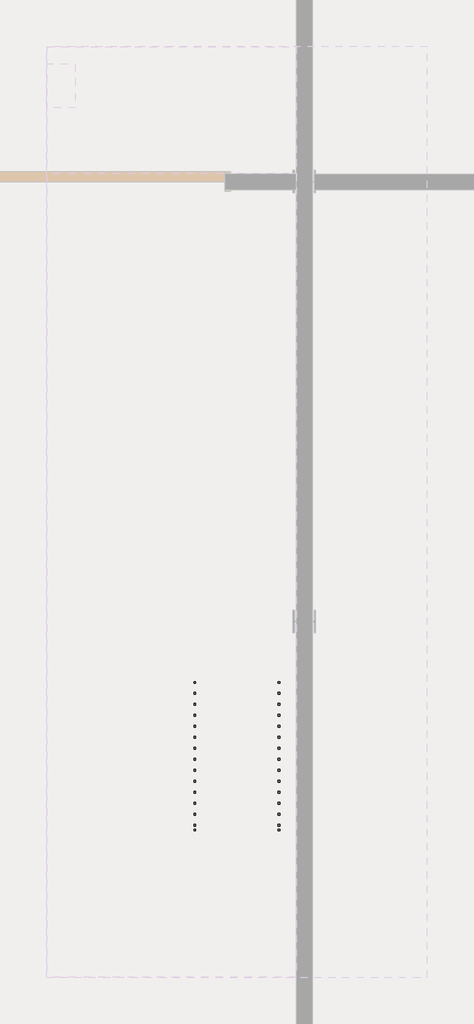
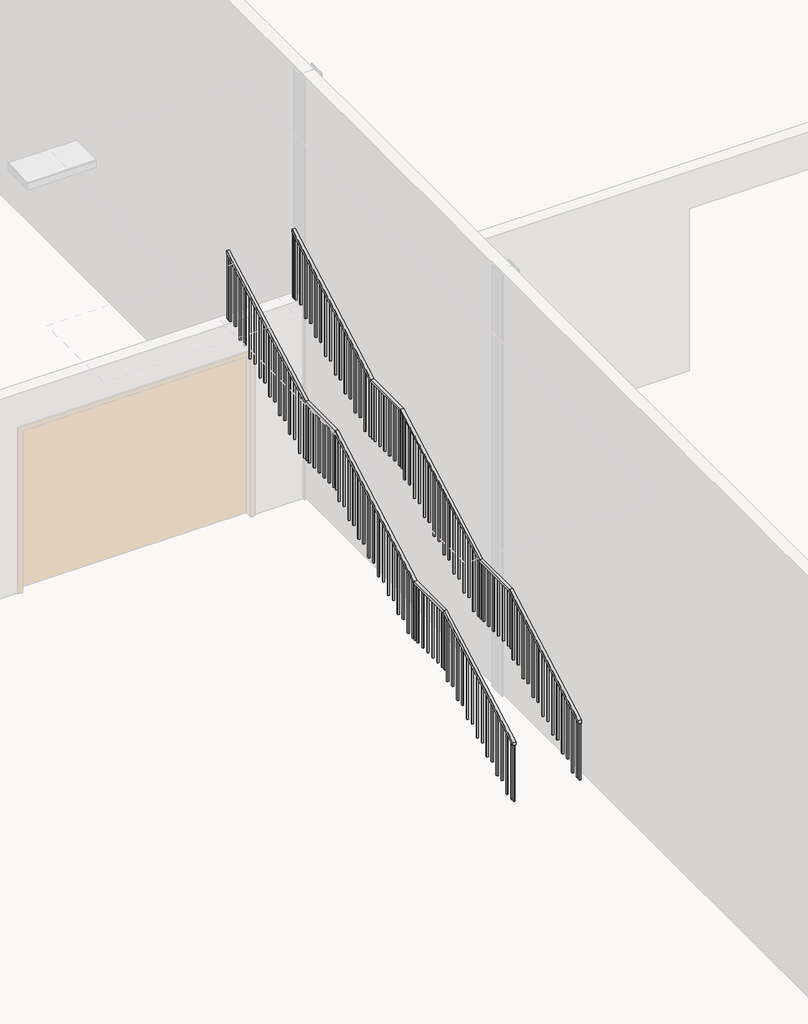
# One storey, part 8 of 13: 2 railings.
"""IFC4 building model written with IfcOpenShell, lengths in millimetres."""

from ifc_helpers import new_model, si_unit, frame, origin, place, context, project, spatial, polyline, outline, extrude, faceted_brep, element, save

model = new_model("IFC4")

# Units and contexts
model_context = context("Model", 3, world=origin())
ifc_project = project(units=[si_unit("LENGTHUNIT", "METRE", prefix="MILLI")], contexts=[model_context])

# Site, building, storey
site = spatial("IfcSite", under=ifc_project)
building = spatial("IfcBuilding", under=site)
storey = spatial("IfcBuildingStorey", under=building, Name="L0 - Ground Floor (Shadows On)", Elevation=0.0)

# Railings
placement = place(None, origin())
element("IfcRailing", 1, ObjectType="1100mm", at=placement, inside=storey, context=model_context, shape_type="SolidModel", body=[
    faceted_brep([(10487.9745537, -13916.6257726, 1266.6666667), (10487.9745537, -13916.6257726, 1209.4687214), (10537.9745537, -13916.6257726, 1209.4687214), (10537.9745537, -13916.6257726, 1266.6666667), (10487.9745537, -11816.6257726, 2433.3333333), (10487.9745537, -11803.6694712, 2383.3333333), (10537.9745537, -11803.6694712, 2383.3333333), (10537.9745537, -11816.6257726, 2433.3333333), (10487.9745537, -10916.6257726, 2433.3333333), (10487.9745537, -10903.6694712, 2383.3333333), (10537.9745537, -10903.6694712, 2383.3333333), (10537.9745537, -10916.6257726, 2433.3333333), (10487.9745537, -8516.6257726, 3766.6666667), (10487.9745537, -8503.6694712, 3716.6666667), (10537.9745537, -8503.6694712, 3716.6666667), (10537.9745537, -8516.6257726, 3766.6666667), (10487.9745537, -7616.6257726, 3766.6666667), (10487.9745537, -7603.6694712, 3716.6666667), (10537.9745537, -7603.6694712, 3716.6666667), (10537.9745537, -7616.6257726, 3766.6666667), (10487.9745537, -5216.6257726, 5100.0), (10537.9745537, -5216.6257726, 5100.0), (10537.9745537, -5216.6257726, 5042.8020548), (10487.9745537, -5216.6257726, 5042.8020548)], [[[0, 1, 2, 3]], [[1, 0, 4, 5]], [[2, 1, 5, 6]], [[3, 2, 6, 7]], [[0, 3, 7, 4]], [[5, 4, 8, 9]], [[6, 5, 9, 10]], [[7, 6, 10, 11]], [[4, 7, 11, 8]], [[9, 8, 12, 13]], [[10, 9, 13, 14]], [[11, 10, 14, 15]], [[8, 11, 15, 12]], [[13, 12, 16, 17]], [[14, 13, 17, 18]], [[15, 14, 18, 19]], [[12, 15, 19, 16]], [[20, 21, 22, 23]], [[17, 16, 20, 23]], [[18, 17, 23, 22]], [[19, 18, 22, 21]], [[16, 19, 21, 20]]]),
    extrude(outline(polyline([(-5304.1257726, 3833.3333333), (-5304.1257726, 4994.1909437), (-5279.1257726, 5008.0798326), (-5279.1257726, 3833.3333333), (-5304.1257726, 3833.3333333)])), frame((10500.4745537, 0.0, 0.0), z_axis=(1.0, 0.0, 0.0), x_axis=(0.0, 1.0, 0.0)), (0.0, 0.0, 1.0), 25.0),
    extrude(outline(polyline([(-5454.1257726, 3833.3333333), (-5454.1257726, 4910.8576103), (-5429.1257726, 4924.7464992), (-5429.1257726, 3833.3333333), (-5454.1257726, 3833.3333333)])), frame((10500.4745537, 0.0, 0.0), z_axis=(1.0, 0.0, 0.0), x_axis=(0.0, 1.0, 0.0)), (0.0, 0.0, 1.0), 25.0),
    extrude(outline(polyline([(-5604.1257726, 3666.6666667), (-5604.1257726, 4827.524277), (-5579.1257726, 4841.4131659), (-5579.1257726, 3666.6666667), (-5604.1257726, 3666.6666667)])), frame((10500.4745537, 0.0, 0.0), z_axis=(1.0, 0.0, 0.0), x_axis=(0.0, 1.0, 0.0)), (0.0, 0.0, 1.0), 25.0),
    extrude(outline(polyline([(-5754.1257726, 3666.6666667), (-5754.1257726, 4744.1909437), (-5729.1257726, 4758.0798326), (-5729.1257726, 3666.6666667), (-5754.1257726, 3666.6666667)])), frame((10500.4745537, 0.0, 0.0), z_axis=(1.0, 0.0, 0.0), x_axis=(0.0, 1.0, 0.0)), (0.0, 0.0, 1.0), 25.0),
    extrude(outline(polyline([(-5904.1257726, 3500.0), (-5904.1257726, 4660.8576103), (-5879.1257726, 4674.7464992), (-5879.1257726, 3500.0), (-5904.1257726, 3500.0)])), frame((10500.4745537, 0.0, 0.0), z_axis=(1.0, 0.0, 0.0), x_axis=(0.0, 1.0, 0.0)), (0.0, 0.0, 1.0), 25.0),
    extrude(outline(polyline([(-6054.1257726, 3500.0), (-6054.1257726, 4577.524277), (-6029.1257726, 4591.4131659), (-6029.1257726, 3500.0), (-6054.1257726, 3500.0)])), frame((10500.4745537, 0.0, 0.0), z_axis=(1.0, 0.0, 0.0), x_axis=(0.0, 1.0, 0.0)), (0.0, 0.0, 1.0), 25.0),
    extrude(outline(polyline([(-6204.1257726, 3333.3333333), (-6204.1257726, 4494.1909437), (-6179.1257726, 4508.0798326), (-6179.1257726, 3333.3333333), (-6204.1257726, 3333.3333333)])), frame((10500.4745537, 0.0, 0.0), z_axis=(1.0, 0.0, 0.0), x_axis=(0.0, 1.0, 0.0)), (0.0, 0.0, 1.0), 25.0),
    extrude(outline(polyline([(-6354.1257726, 3333.3333333), (-6354.1257726, 4410.8576103), (-6329.1257726, 4424.7464992), (-6329.1257726, 3333.3333333), (-6354.1257726, 3333.3333333)])), frame((10500.4745537, 0.0, 0.0), z_axis=(1.0, 0.0, 0.0), x_axis=(0.0, 1.0, 0.0)), (0.0, 0.0, 1.0), 25.0),
    extrude(outline(polyline([(-6504.1257726, 3166.6666667), (-6504.1257726, 4327.524277), (-6479.1257726, 4341.4131659), (-6479.1257726, 3166.6666667), (-6504.1257726, 3166.6666667)])), frame((10500.4745537, 0.0, 0.0), z_axis=(1.0, 0.0, 0.0), x_axis=(0.0, 1.0, 0.0)), (0.0, 0.0, 1.0), 25.0),
    extrude(outline(polyline([(-6654.1257726, 3166.6666667), (-6654.1257726, 4244.1909437), (-6629.1257726, 4258.0798326), (-6629.1257726, 3166.6666667), (-6654.1257726, 3166.6666667)])), frame((10500.4745537, 0.0, 0.0), z_axis=(1.0, 0.0, 0.0), x_axis=(0.0, 1.0, 0.0)), (0.0, 0.0, 1.0), 25.0),
    extrude(outline(polyline([(-6804.1257726, 3000.0), (-6804.1257726, 4160.8576103), (-6779.1257726, 4174.7464992), (-6779.1257726, 3000.0), (-6804.1257726, 3000.0)])), frame((10500.4745537, 0.0, 0.0), z_axis=(1.0, 0.0, 0.0), x_axis=(0.0, 1.0, 0.0)), (0.0, 0.0, 1.0), 25.0),
    extrude(outline(polyline([(-6954.1257726, 3000.0), (-6954.1257726, 4077.524277), (-6929.1257726, 4091.4131659), (-6929.1257726, 3000.0), (-6954.1257726, 3000.0)])), frame((10500.4745537, 0.0, 0.0), z_axis=(1.0, 0.0, 0.0), x_axis=(0.0, 1.0, 0.0)), (0.0, 0.0, 1.0), 25.0),
    extrude(outline(polyline([(-7104.1257726, 2833.3333333), (-7104.1257726, 3994.1909437), (-7079.1257726, 4008.0798326), (-7079.1257726, 2833.3333333), (-7104.1257726, 2833.3333333)])), frame((10500.4745537, 0.0, 0.0), z_axis=(1.0, 0.0, 0.0), x_axis=(0.0, 1.0, 0.0)), (0.0, 0.0, 1.0), 25.0),
    extrude(outline(polyline([(-7254.1257726, 2833.3333333), (-7254.1257726, 3910.8576103), (-7229.1257726, 3924.7464992), (-7229.1257726, 2833.3333333), (-7254.1257726, 2833.3333333)])), frame((10500.4745537, 0.0, 0.0), z_axis=(1.0, 0.0, 0.0), x_axis=(0.0, 1.0, 0.0)), (0.0, 0.0, 1.0), 25.0),
    extrude(outline(polyline([(-7404.1257726, 2666.6666667), (-7404.1257726, 3827.524277), (-7379.1257726, 3841.4131659), (-7379.1257726, 2666.6666667), (-7404.1257726, 2666.6666667)])), frame((10500.4745537, 0.0, 0.0), z_axis=(1.0, 0.0, 0.0), x_axis=(0.0, 1.0, 0.0)), (0.0, 0.0, 1.0), 25.0),
    extrude(outline(polyline([(-7554.1257726, 2666.6666667), (-7554.1257726, 3744.1909437), (-7529.1257726, 3758.0798326), (-7529.1257726, 2666.6666667), (-7554.1257726, 2666.6666667)])), frame((10500.4745537, 0.0, 0.0), z_axis=(1.0, 0.0, 0.0), x_axis=(0.0, 1.0, 0.0)), (0.0, 0.0, 1.0), 25.0),
    extrude(outline(polyline([(10525.4745537, -7704.1257726), (10500.4745537, -7704.1257726), (10500.4745537, -7679.1257726), (10525.4745537, -7679.1257726), (10525.4745537, -7704.1257726)])), frame((0.0, 0.0, 2666.6666667), z_axis=(0.0, 0.0, 1.0), x_axis=(1.0, 0.0, 0.0)), (0.0, 0.0, 1.0), 1050.0),
    extrude(outline(polyline([(10525.4745537, -7854.1257726), (10500.4745537, -7854.1257726), (10500.4745537, -7829.1257726), (10525.4745537, -7829.1257726), (10525.4745537, -7854.1257726)])), frame((0.0, 0.0, 2666.6666667), z_axis=(0.0, 0.0, 1.0), x_axis=(1.0, 0.0, 0.0)), (0.0, 0.0, 1.0), 1050.0),
    extrude(outline(polyline([(10525.4745537, -8004.1257726), (10500.4745537, -8004.1257726), (10500.4745537, -7979.1257726), (10525.4745537, -7979.1257726), (10525.4745537, -8004.1257726)])), frame((0.0, 0.0, 2666.6666667), z_axis=(0.0, 0.0, 1.0), x_axis=(1.0, 0.0, 0.0)), (0.0, 0.0, 1.0), 1050.0),
    extrude(outline(polyline([(10525.4745537, -8154.1257726), (10500.4745537, -8154.1257726), (10500.4745537, -8129.1257726), (10525.4745537, -8129.1257726), (10525.4745537, -8154.1257726)])), frame((0.0, 0.0, 2666.6666667), z_axis=(0.0, 0.0, 1.0), x_axis=(1.0, 0.0, 0.0)), (0.0, 0.0, 1.0), 1050.0),
    extrude(outline(polyline([(10525.4745537, -8304.1257726), (10500.4745537, -8304.1257726), (10500.4745537, -8279.1257726), (10525.4745537, -8279.1257726), (10525.4745537, -8304.1257726)])), frame((0.0, 0.0, 2666.6666667), z_axis=(0.0, 0.0, 1.0), x_axis=(1.0, 0.0, 0.0)), (0.0, 0.0, 1.0), 1050.0),
    extrude(outline(polyline([(10525.4745537, -8454.1257726), (10500.4745537, -8454.1257726), (10500.4745537, -8429.1257726), (10525.4745537, -8429.1257726), (10525.4745537, -8454.1257726)])), frame((0.0, 0.0, 2666.6666667), z_axis=(0.0, 0.0, 1.0), x_axis=(1.0, 0.0, 0.0)), (0.0, 0.0, 1.0), 1050.0),
    extrude(outline(polyline([(-8604.1257726, 2500.0), (-8604.1257726, 3660.8576103), (-8579.1257726, 3674.7464992), (-8579.1257726, 2500.0), (-8604.1257726, 2500.0)])), frame((10500.4745537, 0.0, 0.0), z_axis=(1.0, 0.0, 0.0), x_axis=(0.0, 1.0, 0.0)), (0.0, 0.0, 1.0), 25.0),
    extrude(outline(polyline([(-8754.1257726, 2500.0), (-8754.1257726, 3577.524277), (-8729.1257726, 3591.4131659), (-8729.1257726, 2500.0), (-8754.1257726, 2500.0)])), frame((10500.4745537, 0.0, 0.0), z_axis=(1.0, 0.0, 0.0), x_axis=(0.0, 1.0, 0.0)), (0.0, 0.0, 1.0), 25.0),
    extrude(outline(polyline([(-8904.1257726, 2333.3333333), (-8904.1257726, 3494.1909437), (-8879.1257726, 3508.0798326), (-8879.1257726, 2333.3333333), (-8904.1257726, 2333.3333333)])), frame((10500.4745537, 0.0, 0.0), z_axis=(1.0, 0.0, 0.0), x_axis=(0.0, 1.0, 0.0)), (0.0, 0.0, 1.0), 25.0),
    extrude(outline(polyline([(-9054.1257726, 2333.3333333), (-9054.1257726, 3410.8576103), (-9029.1257726, 3424.7464992), (-9029.1257726, 2333.3333333), (-9054.1257726, 2333.3333333)])), frame((10500.4745537, 0.0, 0.0), z_axis=(1.0, 0.0, 0.0), x_axis=(0.0, 1.0, 0.0)), (0.0, 0.0, 1.0), 25.0),
    extrude(outline(polyline([(-9204.1257726, 2166.6666667), (-9204.1257726, 3327.524277), (-9179.1257726, 3341.4131659), (-9179.1257726, 2166.6666667), (-9204.1257726, 2166.6666667)])), frame((10500.4745537, 0.0, 0.0), z_axis=(1.0, 0.0, 0.0), x_axis=(0.0, 1.0, 0.0)), (0.0, 0.0, 1.0), 25.0),
    extrude(outline(polyline([(-9354.1257726, 2166.6666667), (-9354.1257726, 3244.1909437), (-9329.1257726, 3258.0798326), (-9329.1257726, 2166.6666667), (-9354.1257726, 2166.6666667)])), frame((10500.4745537, 0.0, 0.0), z_axis=(1.0, 0.0, 0.0), x_axis=(0.0, 1.0, 0.0)), (0.0, 0.0, 1.0), 25.0),
    extrude(outline(polyline([(-9504.1257726, 2000.0), (-9504.1257726, 3160.8576103), (-9479.1257726, 3174.7464992), (-9479.1257726, 2000.0), (-9504.1257726, 2000.0)])), frame((10500.4745537, 0.0, 0.0), z_axis=(1.0, 0.0, 0.0), x_axis=(0.0, 1.0, 0.0)), (0.0, 0.0, 1.0), 25.0),
    extrude(outline(polyline([(-9654.1257726, 2000.0), (-9654.1257726, 3077.524277), (-9629.1257726, 3091.4131659), (-9629.1257726, 2000.0), (-9654.1257726, 2000.0)])), frame((10500.4745537, 0.0, 0.0), z_axis=(1.0, 0.0, 0.0), x_axis=(0.0, 1.0, 0.0)), (0.0, 0.0, 1.0), 25.0),
    extrude(outline(polyline([(-9804.1257726, 1833.3333333), (-9804.1257726, 2994.1909437), (-9779.1257726, 3008.0798326), (-9779.1257726, 1833.3333333), (-9804.1257726, 1833.3333333)])), frame((10500.4745537, 0.0, 0.0), z_axis=(1.0, 0.0, 0.0), x_axis=(0.0, 1.0, 0.0)), (0.0, 0.0, 1.0), 25.0),
    extrude(outline(polyline([(-9954.1257726, 1833.3333333), (-9954.1257726, 2910.8576103), (-9929.1257726, 2924.7464992), (-9929.1257726, 1833.3333333), (-9954.1257726, 1833.3333333)])), frame((10500.4745537, 0.0, 0.0), z_axis=(1.0, 0.0, 0.0), x_axis=(0.0, 1.0, 0.0)), (0.0, 0.0, 1.0), 25.0),
    extrude(outline(polyline([(-10104.1257726, 1666.6666667), (-10104.1257726, 2827.524277), (-10079.1257726, 2841.4131659), (-10079.1257726, 1666.6666667), (-10104.1257726, 1666.6666667)])), frame((10500.4745537, 0.0, 0.0), z_axis=(1.0, 0.0, 0.0), x_axis=(0.0, 1.0, 0.0)), (0.0, 0.0, 1.0), 25.0),
    extrude(outline(polyline([(-10254.1257726, 1666.6666667), (-10254.1257726, 2744.1909437), (-10229.1257726, 2758.0798326), (-10229.1257726, 1666.6666667), (-10254.1257726, 1666.6666667)])), frame((10500.4745537, 0.0, 0.0), z_axis=(1.0, 0.0, 0.0), x_axis=(0.0, 1.0, 0.0)), (0.0, 0.0, 1.0), 25.0),
    extrude(outline(polyline([(-10404.1257726, 1500.0), (-10404.1257726, 2660.8576103), (-10379.1257726, 2674.7464992), (-10379.1257726, 1500.0), (-10404.1257726, 1500.0)])), frame((10500.4745537, 0.0, 0.0), z_axis=(1.0, 0.0, 0.0), x_axis=(0.0, 1.0, 0.0)), (0.0, 0.0, 1.0), 25.0),
    extrude(outline(polyline([(-10554.1257726, 1500.0), (-10554.1257726, 2577.524277), (-10529.1257726, 2591.4131659), (-10529.1257726, 1500.0), (-10554.1257726, 1500.0)])), frame((10500.4745537, 0.0, 0.0), z_axis=(1.0, 0.0, 0.0), x_axis=(0.0, 1.0, 0.0)), (0.0, 0.0, 1.0), 25.0),
    extrude(outline(polyline([(-10704.1257726, 1333.3333333), (-10704.1257726, 2494.1909437), (-10679.1257726, 2508.0798326), (-10679.1257726, 1333.3333333), (-10704.1257726, 1333.3333333)])), frame((10500.4745537, 0.0, 0.0), z_axis=(1.0, 0.0, 0.0), x_axis=(0.0, 1.0, 0.0)), (0.0, 0.0, 1.0), 25.0),
    extrude(outline(polyline([(-10854.1257726, 1333.3333333), (-10854.1257726, 2410.8576103), (-10829.1257726, 2424.7464992), (-10829.1257726, 1333.3333333), (-10854.1257726, 1333.3333333)])), frame((10500.4745537, 0.0, 0.0), z_axis=(1.0, 0.0, 0.0), x_axis=(0.0, 1.0, 0.0)), (0.0, 0.0, 1.0), 25.0),
    extrude(outline(polyline([(10525.4745537, -11004.1257726), (10500.4745537, -11004.1257726), (10500.4745537, -10979.1257726), (10525.4745537, -10979.1257726), (10525.4745537, -11004.1257726)])), frame((0.0, 0.0, 1333.3333333), z_axis=(0.0, 0.0, 1.0), x_axis=(1.0, 0.0, 0.0)), (0.0, 0.0, 1.0), 1050.0),
    extrude(outline(polyline([(10525.4745537, -11154.1257726), (10500.4745537, -11154.1257726), (10500.4745537, -11129.1257726), (10525.4745537, -11129.1257726), (10525.4745537, -11154.1257726)])), frame((0.0, 0.0, 1333.3333333), z_axis=(0.0, 0.0, 1.0), x_axis=(1.0, 0.0, 0.0)), (0.0, 0.0, 1.0), 1050.0),
    extrude(outline(polyline([(10525.4745537, -11304.1257726), (10500.4745537, -11304.1257726), (10500.4745537, -11279.1257726), (10525.4745537, -11279.1257726), (10525.4745537, -11304.1257726)])), frame((0.0, 0.0, 1333.3333333), z_axis=(0.0, 0.0, 1.0), x_axis=(1.0, 0.0, 0.0)), (0.0, 0.0, 1.0), 1050.0),
    extrude(outline(polyline([(10525.4745537, -11454.1257726), (10500.4745537, -11454.1257726), (10500.4745537, -11429.1257726), (10525.4745537, -11429.1257726), (10525.4745537, -11454.1257726)])), frame((0.0, 0.0, 1333.3333333), z_axis=(0.0, 0.0, 1.0), x_axis=(1.0, 0.0, 0.0)), (0.0, 0.0, 1.0), 1050.0),
    extrude(outline(polyline([(10525.4745537, -11604.1257726), (10500.4745537, -11604.1257726), (10500.4745537, -11579.1257726), (10525.4745537, -11579.1257726), (10525.4745537, -11604.1257726)])), frame((0.0, 0.0, 1333.3333333), z_axis=(0.0, 0.0, 1.0), x_axis=(1.0, 0.0, 0.0)), (0.0, 0.0, 1.0), 1050.0),
    extrude(outline(polyline([(10525.4745537, -11754.1257726), (10500.4745537, -11754.1257726), (10500.4745537, -11729.1257726), (10525.4745537, -11729.1257726), (10525.4745537, -11754.1257726)])), frame((0.0, 0.0, 1333.3333333), z_axis=(0.0, 0.0, 1.0), x_axis=(1.0, 0.0, 0.0)), (0.0, 0.0, 1.0), 1050.0),
    extrude(outline(polyline([(-11904.1257726, 1166.6666667), (-11904.1257726, 2327.524277), (-11879.1257726, 2341.4131659), (-11879.1257726, 1166.6666667), (-11904.1257726, 1166.6666667)])), frame((10500.4745537, 0.0, 0.0), z_axis=(1.0, 0.0, 0.0), x_axis=(0.0, 1.0, 0.0)), (0.0, 0.0, 1.0), 25.0),
    extrude(outline(polyline([(-12054.1257726, 1166.6666667), (-12054.1257726, 2244.1909437), (-12029.1257726, 2258.0798326), (-12029.1257726, 1166.6666667), (-12054.1257726, 1166.6666667)])), frame((10500.4745537, 0.0, 0.0), z_axis=(1.0, 0.0, 0.0), x_axis=(0.0, 1.0, 0.0)), (0.0, 0.0, 1.0), 25.0),
    extrude(outline(polyline([(-12204.1257726, 1000.0), (-12204.1257726, 2160.8576103), (-12179.1257726, 2174.7464992), (-12179.1257726, 1000.0), (-12204.1257726, 1000.0)])), frame((10500.4745537, 0.0, 0.0), z_axis=(1.0, 0.0, 0.0), x_axis=(0.0, 1.0, 0.0)), (0.0, 0.0, 1.0), 25.0),
    extrude(outline(polyline([(-12354.1257726, 1000.0), (-12354.1257726, 2077.524277), (-12329.1257726, 2091.4131659), (-12329.1257726, 1000.0), (-12354.1257726, 1000.0)])), frame((10500.4745537, 0.0, 0.0), z_axis=(1.0, 0.0, 0.0), x_axis=(0.0, 1.0, 0.0)), (0.0, 0.0, 1.0), 25.0),
    extrude(outline(polyline([(-12504.1257726, 833.3333333), (-12504.1257726, 1994.1909437), (-12479.1257726, 2008.0798326), (-12479.1257726, 833.3333333), (-12504.1257726, 833.3333333)])), frame((10500.4745537, 0.0, 0.0), z_axis=(1.0, 0.0, 0.0), x_axis=(0.0, 1.0, 0.0)), (0.0, 0.0, 1.0), 25.0),
    extrude(outline(polyline([(-12654.1257726, 833.3333333), (-12654.1257726, 1910.8576103), (-12629.1257726, 1924.7464992), (-12629.1257726, 833.3333333), (-12654.1257726, 833.3333333)])), frame((10500.4745537, 0.0, 0.0), z_axis=(1.0, 0.0, 0.0), x_axis=(0.0, 1.0, 0.0)), (0.0, 0.0, 1.0), 25.0),
    extrude(outline(polyline([(-12804.1257726, 666.6666667), (-12804.1257726, 1827.524277), (-12779.1257726, 1841.4131659), (-12779.1257726, 666.6666667), (-12804.1257726, 666.6666667)])), frame((10500.4745537, 0.0, 0.0), z_axis=(1.0, 0.0, 0.0), x_axis=(0.0, 1.0, 0.0)), (0.0, 0.0, 1.0), 25.0),
    extrude(outline(polyline([(-12954.1257726, 666.6666667), (-12954.1257726, 1744.1909437), (-12929.1257726, 1758.0798326), (-12929.1257726, 666.6666667), (-12954.1257726, 666.6666667)])), frame((10500.4745537, 0.0, 0.0), z_axis=(1.0, 0.0, 0.0), x_axis=(0.0, 1.0, 0.0)), (0.0, 0.0, 1.0), 25.0),
    extrude(outline(polyline([(-13104.1257726, 500.0), (-13104.1257726, 1660.8576103), (-13079.1257726, 1674.7464992), (-13079.1257726, 500.0), (-13104.1257726, 500.0)])), frame((10500.4745537, 0.0, 0.0), z_axis=(1.0, 0.0, 0.0), x_axis=(0.0, 1.0, 0.0)), (0.0, 0.0, 1.0), 25.0),
    extrude(outline(polyline([(-13254.1257726, 500.0), (-13254.1257726, 1577.524277), (-13229.1257726, 1591.4131659), (-13229.1257726, 500.0), (-13254.1257726, 500.0)])), frame((10500.4745537, 0.0, 0.0), z_axis=(1.0, 0.0, 0.0), x_axis=(0.0, 1.0, 0.0)), (0.0, 0.0, 1.0), 25.0),
    extrude(outline(polyline([(-13404.1257726, 333.3333333), (-13404.1257726, 1494.1909437), (-13379.1257726, 1508.0798326), (-13379.1257726, 333.3333333), (-13404.1257726, 333.3333333)])), frame((10500.4745537, 0.0, 0.0), z_axis=(1.0, 0.0, 0.0), x_axis=(0.0, 1.0, 0.0)), (0.0, 0.0, 1.0), 25.0),
    extrude(outline(polyline([(-13554.1257726, 333.3333333), (-13554.1257726, 1410.8576103), (-13529.1257726, 1424.7464992), (-13529.1257726, 333.3333333), (-13554.1257726, 333.3333333)])), frame((10500.4745537, 0.0, 0.0), z_axis=(1.0, 0.0, 0.0), x_axis=(0.0, 1.0, 0.0)), (0.0, 0.0, 1.0), 25.0),
    extrude(outline(polyline([(-13704.1257726, 166.6666667), (-13704.1257726, 1327.524277), (-13679.1257726, 1341.4131659), (-13679.1257726, 166.6666667), (-13704.1257726, 166.6666667)])), frame((10500.4745537, 0.0, 0.0), z_axis=(1.0, 0.0, 0.0), x_axis=(0.0, 1.0, 0.0)), (0.0, 0.0, 1.0), 25.0),
    extrude(outline(polyline([(-13854.1257726, 166.6666667), (-13854.1257726, 1244.1909437), (-13829.1257726, 1258.0798326), (-13829.1257726, 166.6666667), (-13854.1257726, 166.6666667)])), frame((10500.4745537, 0.0, 0.0), z_axis=(1.0, 0.0, 0.0), x_axis=(0.0, 1.0, 0.0)), (0.0, 0.0, 1.0), 25.0),
    extrude(outline(polyline([(10525.4745537, -7629.1257726), (10500.4745537, -7629.1257726), (10500.4745537, -7604.1257726), (10525.4745537, -7604.1257726), (10525.4745537, -7629.1257726)])), frame((0.0, 0.0, 2666.6666667), z_axis=(0.0, 0.0, 1.0), x_axis=(1.0, 0.0, 0.0)), (0.0, 0.0, 1.0), 1050.0),
    extrude(outline(polyline([(-8529.1257726, 2666.6666667), (-8529.1257726, 3702.524277), (-8504.1257726, 3716.4131659), (-8504.1257726, 2666.6666667), (-8529.1257726, 2666.6666667)])), frame((10500.4745537, 0.0, 0.0), z_axis=(1.0, 0.0, 0.0), x_axis=(0.0, 1.0, 0.0)), (0.0, 0.0, 1.0), 25.0),
    extrude(outline(polyline([(10525.4745537, -10929.1257726), (10500.4745537, -10929.1257726), (10500.4745537, -10904.1257726), (10525.4745537, -10904.1257726), (10525.4745537, -10929.1257726)])), frame((0.0, 0.0, 1333.3333333), z_axis=(0.0, 0.0, 1.0), x_axis=(1.0, 0.0, 0.0)), (0.0, 0.0, 1.0), 1050.0),
    extrude(outline(polyline([(-11829.1257726, 1333.3333333), (-11829.1257726, 2369.1909437), (-11804.1257726, 2383.0798326), (-11804.1257726, 1333.3333333), (-11829.1257726, 1333.3333333)])), frame((10500.4745537, 0.0, 0.0), z_axis=(1.0, 0.0, 0.0), x_axis=(0.0, 1.0, 0.0)), (0.0, 0.0, 1.0), 25.0),
    extrude(outline(polyline([(-5241.6257726, 3833.3333333), (-5241.6257726, 5028.9131659), (-5216.6257726, 5042.8020548), (-5216.6257726, 3833.3333333), (-5241.6257726, 3833.3333333)])), frame((10500.4745537, 0.0, 0.0), z_axis=(1.0, 0.0, 0.0), x_axis=(0.0, 1.0, 0.0)), (0.0, 0.0, 1.0), 25.0),
    extrude(outline(polyline([(-13916.6257726, 166.6666667), (-13916.6257726, 1209.4687214), (-13891.6257726, 1223.3576103), (-13891.6257726, 166.6666667), (-13916.6257726, 166.6666667)])), frame((10500.4745537, 0.0, 0.0), z_axis=(1.0, 0.0, 0.0), x_axis=(0.0, 1.0, 0.0)), (0.0, 0.0, 1.0), 25.0),
])
element("IfcRailing", 2, ObjectType="1100mm", at=placement, inside=storey, context=model_context, shape_type="SolidModel", body=[
    faceted_brep([(9338.7745537, -13916.6257726, 1266.6666667), (9338.7745537, -13916.6257726, 1209.4687214), (9388.7745537, -13916.6257726, 1209.4687214), (9388.7745537, -13916.6257726, 1266.6666667), (9338.7745537, -11816.6257726, 2433.3333333), (9338.7745537, -11803.6694712, 2383.3333333), (9388.7745537, -11803.6694712, 2383.3333333), (9388.7745537, -11816.6257726, 2433.3333333), (9338.7745537, -10916.6257726, 2433.3333333), (9338.7745537, -10903.6694712, 2383.3333333), (9388.7745537, -10903.6694712, 2383.3333333), (9388.7745537, -10916.6257726, 2433.3333333), (9338.7745537, -8516.6257726, 3766.6666667), (9338.7745537, -8503.6694712, 3716.6666667), (9388.7745537, -8503.6694712, 3716.6666667), (9388.7745537, -8516.6257726, 3766.6666667), (9338.7745537, -7616.6257726, 3766.6666667), (9338.7745537, -7603.6694712, 3716.6666667), (9388.7745537, -7603.6694712, 3716.6666667), (9388.7745537, -7616.6257726, 3766.6666667), (9338.7745537, -5216.6257726, 5100.0), (9388.7745537, -5216.6257726, 5100.0), (9388.7745537, -5216.6257726, 5042.8020548), (9338.7745537, -5216.6257726, 5042.8020548)], [[[0, 1, 2, 3]], [[1, 0, 4, 5]], [[2, 1, 5, 6]], [[3, 2, 6, 7]], [[0, 3, 7, 4]], [[5, 4, 8, 9]], [[6, 5, 9, 10]], [[7, 6, 10, 11]], [[4, 7, 11, 8]], [[9, 8, 12, 13]], [[10, 9, 13, 14]], [[11, 10, 14, 15]], [[8, 11, 15, 12]], [[13, 12, 16, 17]], [[14, 13, 17, 18]], [[15, 14, 18, 19]], [[12, 15, 19, 16]], [[20, 21, 22, 23]], [[17, 16, 20, 23]], [[18, 17, 23, 22]], [[19, 18, 22, 21]], [[16, 19, 21, 20]]]),
    extrude(outline(polyline([(-5304.1257726, 4994.1909437), (-5279.1257726, 5008.0798326), (-5279.1257726, 3833.3333333), (-5304.1257726, 3833.3333333), (-5304.1257726, 4994.1909437)])), frame((9351.2745537, 0.0, 0.0), z_axis=(1.0, 0.0, 0.0), x_axis=(0.0, 1.0, 0.0)), (0.0, 0.0, 1.0), 25.0),
    extrude(outline(polyline([(-5454.1257726, 4910.8576103), (-5429.1257726, 4924.7464992), (-5429.1257726, 3833.3333333), (-5454.1257726, 3833.3333333), (-5454.1257726, 4910.8576103)])), frame((9351.2745537, 0.0, 0.0), z_axis=(1.0, 0.0, 0.0), x_axis=(0.0, 1.0, 0.0)), (0.0, 0.0, 1.0), 25.0),
    extrude(outline(polyline([(-5604.1257726, 4827.524277), (-5579.1257726, 4841.4131659), (-5579.1257726, 3666.6666667), (-5604.1257726, 3666.6666667), (-5604.1257726, 4827.524277)])), frame((9351.2745537, 0.0, 0.0), z_axis=(1.0, 0.0, 0.0), x_axis=(0.0, 1.0, 0.0)), (0.0, 0.0, 1.0), 25.0),
    extrude(outline(polyline([(-5754.1257726, 4744.1909437), (-5729.1257726, 4758.0798326), (-5729.1257726, 3666.6666667), (-5754.1257726, 3666.6666667), (-5754.1257726, 4744.1909437)])), frame((9351.2745537, 0.0, 0.0), z_axis=(1.0, 0.0, 0.0), x_axis=(0.0, 1.0, 0.0)), (0.0, 0.0, 1.0), 25.0),
    extrude(outline(polyline([(-5904.1257726, 4660.8576103), (-5879.1257726, 4674.7464992), (-5879.1257726, 3500.0), (-5904.1257726, 3500.0), (-5904.1257726, 4660.8576103)])), frame((9351.2745537, 0.0, 0.0), z_axis=(1.0, 0.0, 0.0), x_axis=(0.0, 1.0, 0.0)), (0.0, 0.0, 1.0), 25.0),
    extrude(outline(polyline([(-6054.1257726, 4577.524277), (-6029.1257726, 4591.4131659), (-6029.1257726, 3500.0), (-6054.1257726, 3500.0), (-6054.1257726, 4577.524277)])), frame((9351.2745537, 0.0, 0.0), z_axis=(1.0, 0.0, 0.0), x_axis=(0.0, 1.0, 0.0)), (0.0, 0.0, 1.0), 25.0),
    extrude(outline(polyline([(-6204.1257726, 4494.1909437), (-6179.1257726, 4508.0798326), (-6179.1257726, 3333.3333333), (-6204.1257726, 3333.3333333), (-6204.1257726, 4494.1909437)])), frame((9351.2745537, 0.0, 0.0), z_axis=(1.0, 0.0, 0.0), x_axis=(0.0, 1.0, 0.0)), (0.0, 0.0, 1.0), 25.0),
    extrude(outline(polyline([(-6354.1257726, 4410.8576103), (-6329.1257726, 4424.7464992), (-6329.1257726, 3333.3333333), (-6354.1257726, 3333.3333333), (-6354.1257726, 4410.8576103)])), frame((9351.2745537, 0.0, 0.0), z_axis=(1.0, 0.0, 0.0), x_axis=(0.0, 1.0, 0.0)), (0.0, 0.0, 1.0), 25.0),
    extrude(outline(polyline([(-6504.1257726, 4327.524277), (-6479.1257726, 4341.4131659), (-6479.1257726, 3166.6666667), (-6504.1257726, 3166.6666667), (-6504.1257726, 4327.524277)])), frame((9351.2745537, 0.0, 0.0), z_axis=(1.0, 0.0, 0.0), x_axis=(0.0, 1.0, 0.0)), (0.0, 0.0, 1.0), 25.0),
    extrude(outline(polyline([(-6654.1257726, 4244.1909437), (-6629.1257726, 4258.0798326), (-6629.1257726, 3166.6666667), (-6654.1257726, 3166.6666667), (-6654.1257726, 4244.1909437)])), frame((9351.2745537, 0.0, 0.0), z_axis=(1.0, 0.0, 0.0), x_axis=(0.0, 1.0, 0.0)), (0.0, 0.0, 1.0), 25.0),
    extrude(outline(polyline([(-6804.1257726, 4160.8576103), (-6779.1257726, 4174.7464992), (-6779.1257726, 3000.0), (-6804.1257726, 3000.0), (-6804.1257726, 4160.8576103)])), frame((9351.2745537, 0.0, 0.0), z_axis=(1.0, 0.0, 0.0), x_axis=(0.0, 1.0, 0.0)), (0.0, 0.0, 1.0), 25.0),
    extrude(outline(polyline([(-6954.1257726, 4077.524277), (-6929.1257726, 4091.4131659), (-6929.1257726, 3000.0), (-6954.1257726, 3000.0), (-6954.1257726, 4077.524277)])), frame((9351.2745537, 0.0, 0.0), z_axis=(1.0, 0.0, 0.0), x_axis=(0.0, 1.0, 0.0)), (0.0, 0.0, 1.0), 25.0),
    extrude(outline(polyline([(-7104.1257726, 3994.1909437), (-7079.1257726, 4008.0798326), (-7079.1257726, 2833.3333333), (-7104.1257726, 2833.3333333), (-7104.1257726, 3994.1909437)])), frame((9351.2745537, 0.0, 0.0), z_axis=(1.0, 0.0, 0.0), x_axis=(0.0, 1.0, 0.0)), (0.0, 0.0, 1.0), 25.0),
    extrude(outline(polyline([(-7254.1257726, 3910.8576103), (-7229.1257726, 3924.7464992), (-7229.1257726, 2833.3333333), (-7254.1257726, 2833.3333333), (-7254.1257726, 3910.8576103)])), frame((9351.2745537, 0.0, 0.0), z_axis=(1.0, 0.0, 0.0), x_axis=(0.0, 1.0, 0.0)), (0.0, 0.0, 1.0), 25.0),
    extrude(outline(polyline([(-7404.1257726, 3827.524277), (-7379.1257726, 3841.4131659), (-7379.1257726, 2666.6666667), (-7404.1257726, 2666.6666667), (-7404.1257726, 3827.524277)])), frame((9351.2745537, 0.0, 0.0), z_axis=(1.0, 0.0, 0.0), x_axis=(0.0, 1.0, 0.0)), (0.0, 0.0, 1.0), 25.0),
    extrude(outline(polyline([(-7554.1257726, 3744.1909437), (-7529.1257726, 3758.0798326), (-7529.1257726, 2666.6666667), (-7554.1257726, 2666.6666667), (-7554.1257726, 3744.1909437)])), frame((9351.2745537, 0.0, 0.0), z_axis=(1.0, 0.0, 0.0), x_axis=(0.0, 1.0, 0.0)), (0.0, 0.0, 1.0), 25.0),
    extrude(outline(polyline([(9351.2745537, -7704.1257726), (9351.2745537, -7679.1257726), (9376.2745537, -7679.1257726), (9376.2745537, -7704.1257726), (9351.2745537, -7704.1257726)])), frame((0.0, 0.0, 2666.6666667), z_axis=(0.0, 0.0, 1.0), x_axis=(1.0, 0.0, 0.0)), (0.0, 0.0, 1.0), 1050.0),
    extrude(outline(polyline([(9351.2745537, -7854.1257726), (9351.2745537, -7829.1257726), (9376.2745537, -7829.1257726), (9376.2745537, -7854.1257726), (9351.2745537, -7854.1257726)])), frame((0.0, 0.0, 2666.6666667), z_axis=(0.0, 0.0, 1.0), x_axis=(1.0, 0.0, 0.0)), (0.0, 0.0, 1.0), 1050.0),
    extrude(outline(polyline([(9351.2745537, -8004.1257726), (9351.2745537, -7979.1257726), (9376.2745537, -7979.1257726), (9376.2745537, -8004.1257726), (9351.2745537, -8004.1257726)])), frame((0.0, 0.0, 2666.6666667), z_axis=(0.0, 0.0, 1.0), x_axis=(1.0, 0.0, 0.0)), (0.0, 0.0, 1.0), 1050.0),
    extrude(outline(polyline([(9351.2745537, -8154.1257726), (9351.2745537, -8129.1257726), (9376.2745537, -8129.1257726), (9376.2745537, -8154.1257726), (9351.2745537, -8154.1257726)])), frame((0.0, 0.0, 2666.6666667), z_axis=(0.0, 0.0, 1.0), x_axis=(1.0, 0.0, 0.0)), (0.0, 0.0, 1.0), 1050.0),
    extrude(outline(polyline([(9351.2745537, -8304.1257726), (9351.2745537, -8279.1257726), (9376.2745537, -8279.1257726), (9376.2745537, -8304.1257726), (9351.2745537, -8304.1257726)])), frame((0.0, 0.0, 2666.6666667), z_axis=(0.0, 0.0, 1.0), x_axis=(1.0, 0.0, 0.0)), (0.0, 0.0, 1.0), 1050.0),
    extrude(outline(polyline([(9351.2745537, -8454.1257726), (9351.2745537, -8429.1257726), (9376.2745537, -8429.1257726), (9376.2745537, -8454.1257726), (9351.2745537, -8454.1257726)])), frame((0.0, 0.0, 2666.6666667), z_axis=(0.0, 0.0, 1.0), x_axis=(1.0, 0.0, 0.0)), (0.0, 0.0, 1.0), 1050.0),
    extrude(outline(polyline([(-8604.1257726, 3660.8576103), (-8579.1257726, 3674.7464992), (-8579.1257726, 2500.0), (-8604.1257726, 2500.0), (-8604.1257726, 3660.8576103)])), frame((9351.2745537, 0.0, 0.0), z_axis=(1.0, 0.0, 0.0), x_axis=(0.0, 1.0, 0.0)), (0.0, 0.0, 1.0), 25.0),
    extrude(outline(polyline([(-8754.1257726, 3577.524277), (-8729.1257726, 3591.4131659), (-8729.1257726, 2500.0), (-8754.1257726, 2500.0), (-8754.1257726, 3577.524277)])), frame((9351.2745537, 0.0, 0.0), z_axis=(1.0, 0.0, 0.0), x_axis=(0.0, 1.0, 0.0)), (0.0, 0.0, 1.0), 25.0),
    extrude(outline(polyline([(-8904.1257726, 3494.1909437), (-8879.1257726, 3508.0798326), (-8879.1257726, 2333.3333333), (-8904.1257726, 2333.3333333), (-8904.1257726, 3494.1909437)])), frame((9351.2745537, 0.0, 0.0), z_axis=(1.0, 0.0, 0.0), x_axis=(0.0, 1.0, 0.0)), (0.0, 0.0, 1.0), 25.0),
    extrude(outline(polyline([(-9054.1257726, 3410.8576103), (-9029.1257726, 3424.7464992), (-9029.1257726, 2333.3333333), (-9054.1257726, 2333.3333333), (-9054.1257726, 3410.8576103)])), frame((9351.2745537, 0.0, 0.0), z_axis=(1.0, 0.0, 0.0), x_axis=(0.0, 1.0, 0.0)), (0.0, 0.0, 1.0), 25.0),
    extrude(outline(polyline([(-9204.1257726, 3327.524277), (-9179.1257726, 3341.4131659), (-9179.1257726, 2166.6666667), (-9204.1257726, 2166.6666667), (-9204.1257726, 3327.524277)])), frame((9351.2745537, 0.0, 0.0), z_axis=(1.0, 0.0, 0.0), x_axis=(0.0, 1.0, 0.0)), (0.0, 0.0, 1.0), 25.0),
    extrude(outline(polyline([(-9354.1257726, 3244.1909437), (-9329.1257726, 3258.0798326), (-9329.1257726, 2166.6666667), (-9354.1257726, 2166.6666667), (-9354.1257726, 3244.1909437)])), frame((9351.2745537, 0.0, 0.0), z_axis=(1.0, 0.0, 0.0), x_axis=(0.0, 1.0, 0.0)), (0.0, 0.0, 1.0), 25.0),
    extrude(outline(polyline([(-9504.1257726, 3160.8576103), (-9479.1257726, 3174.7464992), (-9479.1257726, 2000.0), (-9504.1257726, 2000.0), (-9504.1257726, 3160.8576103)])), frame((9351.2745537, 0.0, 0.0), z_axis=(1.0, 0.0, 0.0), x_axis=(0.0, 1.0, 0.0)), (0.0, 0.0, 1.0), 25.0),
    extrude(outline(polyline([(-9654.1257726, 3077.524277), (-9629.1257726, 3091.4131659), (-9629.1257726, 2000.0), (-9654.1257726, 2000.0), (-9654.1257726, 3077.524277)])), frame((9351.2745537, 0.0, 0.0), z_axis=(1.0, 0.0, 0.0), x_axis=(0.0, 1.0, 0.0)), (0.0, 0.0, 1.0), 25.0),
    extrude(outline(polyline([(-9804.1257726, 2994.1909437), (-9779.1257726, 3008.0798326), (-9779.1257726, 1833.3333333), (-9804.1257726, 1833.3333333), (-9804.1257726, 2994.1909437)])), frame((9351.2745537, 0.0, 0.0), z_axis=(1.0, 0.0, 0.0), x_axis=(0.0, 1.0, 0.0)), (0.0, 0.0, 1.0), 25.0),
    extrude(outline(polyline([(-9954.1257726, 2910.8576103), (-9929.1257726, 2924.7464992), (-9929.1257726, 1833.3333333), (-9954.1257726, 1833.3333333), (-9954.1257726, 2910.8576103)])), frame((9351.2745537, 0.0, 0.0), z_axis=(1.0, 0.0, 0.0), x_axis=(0.0, 1.0, 0.0)), (0.0, 0.0, 1.0), 25.0),
    extrude(outline(polyline([(-10104.1257726, 2827.524277), (-10079.1257726, 2841.4131659), (-10079.1257726, 1666.6666667), (-10104.1257726, 1666.6666667), (-10104.1257726, 2827.524277)])), frame((9351.2745537, 0.0, 0.0), z_axis=(1.0, 0.0, 0.0), x_axis=(0.0, 1.0, 0.0)), (0.0, 0.0, 1.0), 25.0),
    extrude(outline(polyline([(-10254.1257726, 2744.1909437), (-10229.1257726, 2758.0798326), (-10229.1257726, 1666.6666667), (-10254.1257726, 1666.6666667), (-10254.1257726, 2744.1909437)])), frame((9351.2745537, 0.0, 0.0), z_axis=(1.0, 0.0, 0.0), x_axis=(0.0, 1.0, 0.0)), (0.0, 0.0, 1.0), 25.0),
    extrude(outline(polyline([(-10404.1257726, 2660.8576103), (-10379.1257726, 2674.7464992), (-10379.1257726, 1500.0), (-10404.1257726, 1500.0), (-10404.1257726, 2660.8576103)])), frame((9351.2745537, 0.0, 0.0), z_axis=(1.0, 0.0, 0.0), x_axis=(0.0, 1.0, 0.0)), (0.0, 0.0, 1.0), 25.0),
    extrude(outline(polyline([(-10554.1257726, 2577.524277), (-10529.1257726, 2591.4131659), (-10529.1257726, 1500.0), (-10554.1257726, 1500.0), (-10554.1257726, 2577.524277)])), frame((9351.2745537, 0.0, 0.0), z_axis=(1.0, 0.0, 0.0), x_axis=(0.0, 1.0, 0.0)), (0.0, 0.0, 1.0), 25.0),
    extrude(outline(polyline([(-10704.1257726, 2494.1909437), (-10679.1257726, 2508.0798326), (-10679.1257726, 1333.3333333), (-10704.1257726, 1333.3333333), (-10704.1257726, 2494.1909437)])), frame((9351.2745537, 0.0, 0.0), z_axis=(1.0, 0.0, 0.0), x_axis=(0.0, 1.0, 0.0)), (0.0, 0.0, 1.0), 25.0),
    extrude(outline(polyline([(-10854.1257726, 2410.8576103), (-10829.1257726, 2424.7464992), (-10829.1257726, 1333.3333333), (-10854.1257726, 1333.3333333), (-10854.1257726, 2410.8576103)])), frame((9351.2745537, 0.0, 0.0), z_axis=(1.0, 0.0, 0.0), x_axis=(0.0, 1.0, 0.0)), (0.0, 0.0, 1.0), 25.0),
    extrude(outline(polyline([(9351.2745537, -11004.1257726), (9351.2745537, -10979.1257726), (9376.2745537, -10979.1257726), (9376.2745537, -11004.1257726), (9351.2745537, -11004.1257726)])), frame((0.0, 0.0, 1333.3333333), z_axis=(0.0, 0.0, 1.0), x_axis=(1.0, 0.0, 0.0)), (0.0, 0.0, 1.0), 1050.0),
    extrude(outline(polyline([(9351.2745537, -11154.1257726), (9351.2745537, -11129.1257726), (9376.2745537, -11129.1257726), (9376.2745537, -11154.1257726), (9351.2745537, -11154.1257726)])), frame((0.0, 0.0, 1333.3333333), z_axis=(0.0, 0.0, 1.0), x_axis=(1.0, 0.0, 0.0)), (0.0, 0.0, 1.0), 1050.0),
    extrude(outline(polyline([(9351.2745537, -11304.1257726), (9351.2745537, -11279.1257726), (9376.2745537, -11279.1257726), (9376.2745537, -11304.1257726), (9351.2745537, -11304.1257726)])), frame((0.0, 0.0, 1333.3333333), z_axis=(0.0, 0.0, 1.0), x_axis=(1.0, 0.0, 0.0)), (0.0, 0.0, 1.0), 1050.0),
    extrude(outline(polyline([(9351.2745537, -11454.1257726), (9351.2745537, -11429.1257726), (9376.2745537, -11429.1257726), (9376.2745537, -11454.1257726), (9351.2745537, -11454.1257726)])), frame((0.0, 0.0, 1333.3333333), z_axis=(0.0, 0.0, 1.0), x_axis=(1.0, 0.0, 0.0)), (0.0, 0.0, 1.0), 1050.0),
    extrude(outline(polyline([(9351.2745537, -11604.1257726), (9351.2745537, -11579.1257726), (9376.2745537, -11579.1257726), (9376.2745537, -11604.1257726), (9351.2745537, -11604.1257726)])), frame((0.0, 0.0, 1333.3333333), z_axis=(0.0, 0.0, 1.0), x_axis=(1.0, 0.0, 0.0)), (0.0, 0.0, 1.0), 1050.0),
    extrude(outline(polyline([(9351.2745537, -11754.1257726), (9351.2745537, -11729.1257726), (9376.2745537, -11729.1257726), (9376.2745537, -11754.1257726), (9351.2745537, -11754.1257726)])), frame((0.0, 0.0, 1333.3333333), z_axis=(0.0, 0.0, 1.0), x_axis=(1.0, 0.0, 0.0)), (0.0, 0.0, 1.0), 1050.0),
    extrude(outline(polyline([(-11904.1257726, 2327.524277), (-11879.1257726, 2341.4131659), (-11879.1257726, 1166.6666667), (-11904.1257726, 1166.6666667), (-11904.1257726, 2327.524277)])), frame((9351.2745537, 0.0, 0.0), z_axis=(1.0, 0.0, 0.0), x_axis=(0.0, 1.0, 0.0)), (0.0, 0.0, 1.0), 25.0),
    extrude(outline(polyline([(-12054.1257726, 2244.1909437), (-12029.1257726, 2258.0798326), (-12029.1257726, 1166.6666667), (-12054.1257726, 1166.6666667), (-12054.1257726, 2244.1909437)])), frame((9351.2745537, 0.0, 0.0), z_axis=(1.0, 0.0, 0.0), x_axis=(0.0, 1.0, 0.0)), (0.0, 0.0, 1.0), 25.0),
    extrude(outline(polyline([(-12204.1257726, 2160.8576103), (-12179.1257726, 2174.7464992), (-12179.1257726, 1000.0), (-12204.1257726, 1000.0), (-12204.1257726, 2160.8576103)])), frame((9351.2745537, 0.0, 0.0), z_axis=(1.0, 0.0, 0.0), x_axis=(0.0, 1.0, 0.0)), (0.0, 0.0, 1.0), 25.0),
    extrude(outline(polyline([(-12354.1257726, 2077.524277), (-12329.1257726, 2091.4131659), (-12329.1257726, 1000.0), (-12354.1257726, 1000.0), (-12354.1257726, 2077.524277)])), frame((9351.2745537, 0.0, 0.0), z_axis=(1.0, 0.0, 0.0), x_axis=(0.0, 1.0, 0.0)), (0.0, 0.0, 1.0), 25.0),
    extrude(outline(polyline([(-12504.1257726, 1994.1909437), (-12479.1257726, 2008.0798326), (-12479.1257726, 833.3333333), (-12504.1257726, 833.3333333), (-12504.1257726, 1994.1909437)])), frame((9351.2745537, 0.0, 0.0), z_axis=(1.0, 0.0, 0.0), x_axis=(0.0, 1.0, 0.0)), (0.0, 0.0, 1.0), 25.0),
    extrude(outline(polyline([(-12654.1257726, 1910.8576103), (-12629.1257726, 1924.7464992), (-12629.1257726, 833.3333333), (-12654.1257726, 833.3333333), (-12654.1257726, 1910.8576103)])), frame((9351.2745537, 0.0, 0.0), z_axis=(1.0, 0.0, 0.0), x_axis=(0.0, 1.0, 0.0)), (0.0, 0.0, 1.0), 25.0),
    extrude(outline(polyline([(-12804.1257726, 1827.524277), (-12779.1257726, 1841.4131659), (-12779.1257726, 666.6666667), (-12804.1257726, 666.6666667), (-12804.1257726, 1827.524277)])), frame((9351.2745537, 0.0, 0.0), z_axis=(1.0, 0.0, 0.0), x_axis=(0.0, 1.0, 0.0)), (0.0, 0.0, 1.0), 25.0),
    extrude(outline(polyline([(-12954.1257726, 1744.1909437), (-12929.1257726, 1758.0798326), (-12929.1257726, 666.6666667), (-12954.1257726, 666.6666667), (-12954.1257726, 1744.1909437)])), frame((9351.2745537, 0.0, 0.0), z_axis=(1.0, 0.0, 0.0), x_axis=(0.0, 1.0, 0.0)), (0.0, 0.0, 1.0), 25.0),
    extrude(outline(polyline([(-13104.1257726, 1660.8576103), (-13079.1257726, 1674.7464992), (-13079.1257726, 500.0), (-13104.1257726, 500.0), (-13104.1257726, 1660.8576103)])), frame((9351.2745537, 0.0, 0.0), z_axis=(1.0, 0.0, 0.0), x_axis=(0.0, 1.0, 0.0)), (0.0, 0.0, 1.0), 25.0),
    extrude(outline(polyline([(-13254.1257726, 1577.524277), (-13229.1257726, 1591.4131659), (-13229.1257726, 500.0), (-13254.1257726, 500.0), (-13254.1257726, 1577.524277)])), frame((9351.2745537, 0.0, 0.0), z_axis=(1.0, 0.0, 0.0), x_axis=(0.0, 1.0, 0.0)), (0.0, 0.0, 1.0), 25.0),
    extrude(outline(polyline([(-13404.1257726, 1494.1909437), (-13379.1257726, 1508.0798326), (-13379.1257726, 333.3333333), (-13404.1257726, 333.3333333), (-13404.1257726, 1494.1909437)])), frame((9351.2745537, 0.0, 0.0), z_axis=(1.0, 0.0, 0.0), x_axis=(0.0, 1.0, 0.0)), (0.0, 0.0, 1.0), 25.0),
    extrude(outline(polyline([(-13554.1257726, 1410.8576103), (-13529.1257726, 1424.7464992), (-13529.1257726, 333.3333333), (-13554.1257726, 333.3333333), (-13554.1257726, 1410.8576103)])), frame((9351.2745537, 0.0, 0.0), z_axis=(1.0, 0.0, 0.0), x_axis=(0.0, 1.0, 0.0)), (0.0, 0.0, 1.0), 25.0),
    extrude(outline(polyline([(-13704.1257726, 1327.524277), (-13679.1257726, 1341.4131659), (-13679.1257726, 166.6666667), (-13704.1257726, 166.6666667), (-13704.1257726, 1327.524277)])), frame((9351.2745537, 0.0, 0.0), z_axis=(1.0, 0.0, 0.0), x_axis=(0.0, 1.0, 0.0)), (0.0, 0.0, 1.0), 25.0),
    extrude(outline(polyline([(-13854.1257726, 1244.1909437), (-13829.1257726, 1258.0798326), (-13829.1257726, 166.6666667), (-13854.1257726, 166.6666667), (-13854.1257726, 1244.1909437)])), frame((9351.2745537, 0.0, 0.0), z_axis=(1.0, 0.0, 0.0), x_axis=(0.0, 1.0, 0.0)), (0.0, 0.0, 1.0), 25.0),
    extrude(outline(polyline([(9351.2745537, -7629.1257726), (9351.2745537, -7604.1257726), (9376.2745537, -7604.1257726), (9376.2745537, -7629.1257726), (9351.2745537, -7629.1257726)])), frame((0.0, 0.0, 2666.6666667), z_axis=(0.0, 0.0, 1.0), x_axis=(1.0, 0.0, 0.0)), (0.0, 0.0, 1.0), 1050.0),
    extrude(outline(polyline([(-8529.1257726, 3702.524277), (-8504.1257726, 3716.4131659), (-8504.1257726, 2666.6666667), (-8529.1257726, 2666.6666667), (-8529.1257726, 3702.524277)])), frame((9351.2745537, 0.0, 0.0), z_axis=(1.0, 0.0, 0.0), x_axis=(0.0, 1.0, 0.0)), (0.0, 0.0, 1.0), 25.0),
    extrude(outline(polyline([(9351.2745537, -10929.1257726), (9351.2745537, -10904.1257726), (9376.2745537, -10904.1257726), (9376.2745537, -10929.1257726), (9351.2745537, -10929.1257726)])), frame((0.0, 0.0, 1333.3333333), z_axis=(0.0, 0.0, 1.0), x_axis=(1.0, 0.0, 0.0)), (0.0, 0.0, 1.0), 1050.0),
    extrude(outline(polyline([(-11829.1257726, 2369.1909437), (-11804.1257726, 2383.0798326), (-11804.1257726, 1333.3333333), (-11829.1257726, 1333.3333333), (-11829.1257726, 2369.1909437)])), frame((9351.2745537, 0.0, 0.0), z_axis=(1.0, 0.0, 0.0), x_axis=(0.0, 1.0, 0.0)), (0.0, 0.0, 1.0), 25.0),
    extrude(outline(polyline([(-5241.6257726, 5028.9131659), (-5216.6257726, 5042.8020548), (-5216.6257726, 3833.3333333), (-5241.6257726, 3833.3333333), (-5241.6257726, 5028.9131659)])), frame((9351.2745537, 0.0, 0.0), z_axis=(1.0, 0.0, 0.0), x_axis=(0.0, 1.0, 0.0)), (0.0, 0.0, 1.0), 25.0),
    extrude(outline(polyline([(-13916.6257726, 1209.4687214), (-13891.6257726, 1223.3576103), (-13891.6257726, 166.6666667), (-13916.6257726, 166.6666667), (-13916.6257726, 1209.4687214)])), frame((9351.2745537, 0.0, 0.0), z_axis=(1.0, 0.0, 0.0), x_axis=(0.0, 1.0, 0.0)), (0.0, 0.0, 1.0), 25.0),
])

save(model, "model.ifc")

# Revit data of these elements
# Type "1100mm"
#   built-in parameter 1008612 = 0.019685 (stored number, unit not read)
#   built-in parameter 1008611 = 0.019685 (stored number, unit not read)
#   built-in parameter 1008609 = 0.902231 (stored number, unit not read)
#   built-in parameter 1008604 = 0.19685 (stored number, unit not read)
#   built-in parameter 1008603 = 0.164042 (stored number, unit not read)
#   Railing Height = 1100 mm
#   built-in parameter 1008630 = 2
#   built-in parameter 1008610 = 2
#   built-in parameter 1008608 = 1
#   built-in parameter 1008618 = Baluster - Square : 25mm
# Elements 1, 2 (IfcRailing, "1100mm")
#   Phase Created = New Construction
